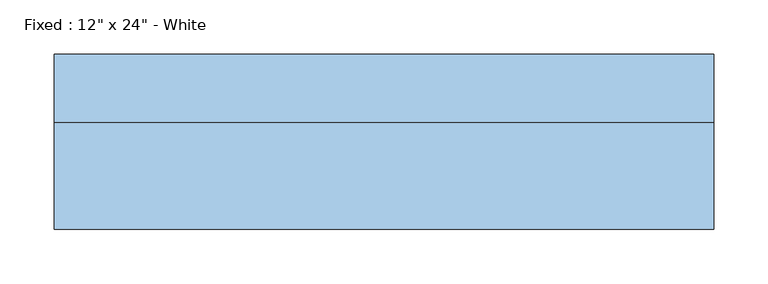
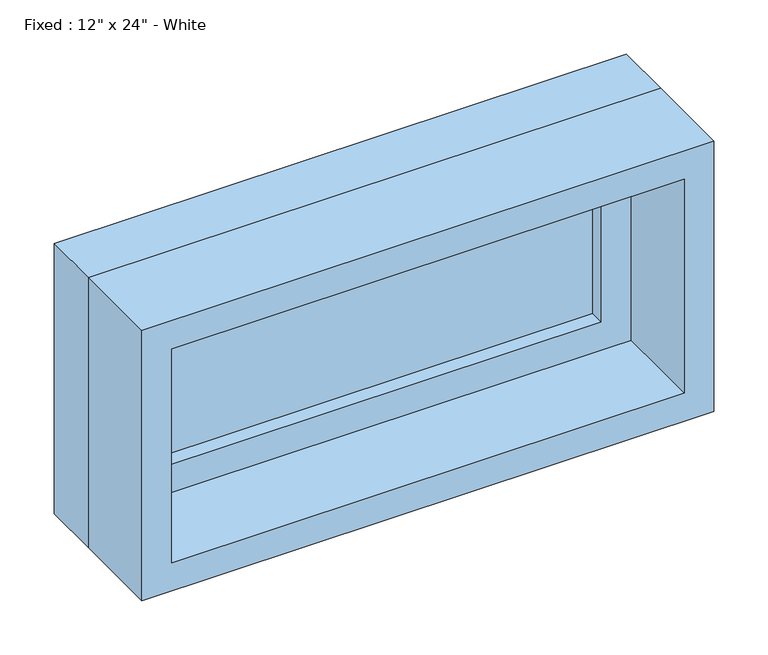
"""IFC4 building model written with IfcOpenShell, lengths in millimetres: window geometry."""

from ifc_helpers import new_model, si_unit, frame, origin, place, context, project, spatial, polyline, outline, extrude, source, transform, mapped, element, save


def window_760927d8(model_context):
    return source(origin(), model_context, "Body", "SweptSolid", [
        extrude(outline(polyline([(203.2, 33.3375), (-279.4, 33.3375), (-279.4, 46.0375), (203.2, 46.0375), (203.2, 33.3375)])), frame((0.0, 0.0, 977.9), z_axis=(0.0, 0.0, 1.0), x_axis=(1.0, 0.0, 0.0)), (0.0, 0.0, 1.0), 177.8),
        extrude(outline(polyline([(1200.15, -323.85), (933.45, -323.85), (933.45, 247.65), (1200.15, 247.65), (1200.15, -323.85)]), holes=[polyline([(1155.7, -279.4), (1155.7, 203.2), (977.9, 203.2), (977.9, -279.4), (1155.7, -279.4)])]), frame((0.0, 17.4625, 0.0), z_axis=(0.0, 1.0, 0.0), x_axis=(0.0, 0.0, 1.0)), (0.0, 0.0, 1.0), 44.45),
        extrude(outline(polyline([(1219.2, -342.9), (914.4, -342.9), (914.4, 266.7), (1219.2, 266.7), (1219.2, -342.9)]), holes=[polyline([(1187.45, -311.15), (1187.45, 234.95), (946.15, 234.95), (946.15, -311.15), (1187.45, -311.15)])]), frame((0.0, -80.9625, 0.0), z_axis=(0.0, 1.0, 0.0), x_axis=(0.0, 0.0, 1.0)), (0.0, 0.0, 1.0), 98.425),
        extrude(outline(polyline([(1219.2, 266.7), (1219.2, -342.9), (914.4, -342.9), (914.4, 266.7), (1219.2, 266.7)]), holes=[polyline([(1200.15, 247.65), (933.45, 247.65), (933.45, -323.85), (1200.15, -323.85), (1200.15, 247.65)])]), frame((0.0, 17.4625, 0.0), z_axis=(0.0, 1.0, 0.0), x_axis=(0.0, 0.0, 1.0)), (0.0, 0.0, 1.0), 63.5),
    ])


if __name__ == "__main__":
    model = new_model("IFC4")
    model_context = context("Model", 3, world=origin())
    ifc_project = project(units=[si_unit("LENGTHUNIT", "METRE", prefix="MILLI")], contexts=[model_context])
    site = spatial("IfcSite", under=ifc_project)
    building = spatial("IfcBuilding", under=site)
    placement = place(None, origin())
    window_shape = window_760927d8(model_context)
    element("IfcWindow", 1, ObjectType="Fixed : 12\" x 24\" - White", at=placement, inside=building, context=model_context, shape_type="MappedRepresentation", body=[
        mapped(window_shape, transform((0.0, 0.0, 0.0), x_axis=(1.0, 0.0, 0.0), y_axis=(0.0, 1.0, 0.0), z_axis=(0.0, 0.0, 1.0))),
    ])
    save(model, "model.ifc")

# Revit data of these elements
# Type "Fixed : 12\" x 24\" - White"
#   Type Mark = "75"
#   Construction Type Id = "GSP4R"
#   Assembly Code = "B2020100"
#   Analytic Construction = "1/8 in Pilkington single glazing"
#   Visual Light Transmittance = 0.9
#   Solar Heat Gain Coefficient = 0.78
#   Heat Transfer Coefficient (U) = 3.6886 W/(m²·K)
#   Height = 1' - 0"
#   Default Sill Height = 3' - 0"
#   Width = 2' - 0"
#   Window Inset = 0' - 0 3/4"
#   COBie.Type = no
#   Glass Pane Material = Glass
#   Sash Material = Sash - White
#   Wall Closure = (empty or 0)
# Element 1 (IfcWindow, "Fixed : 12\" x 24\" - White")
#   Materials on its faces: "Sash - White", "Glass"
# Materials
#   "Glass": class "Glass", colour RGB 0 128 192, transparency 0.75, Description = "Soda Lime Glass", Cost = 0
#   "Sash - White": class "Wood", colour RGB 255 255 255, transparency 0, Cost = 0
